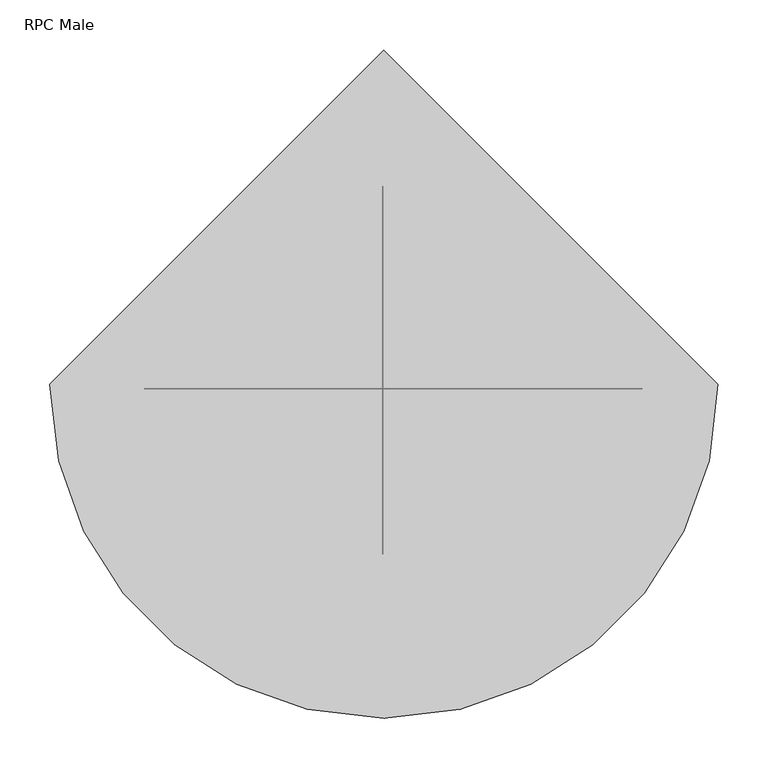
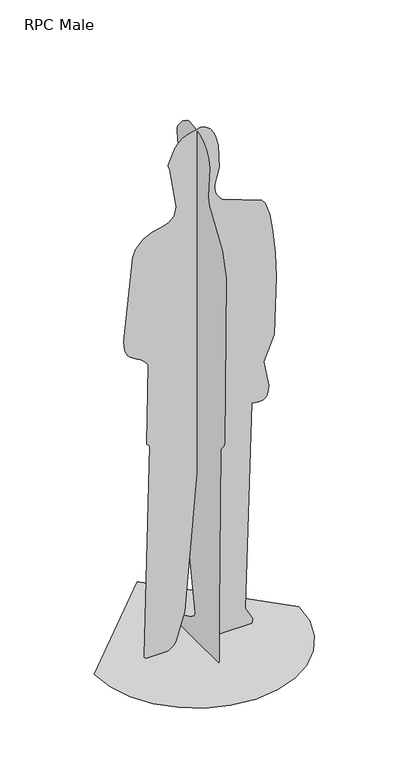
"""IFC4 building model written with IfcOpenShell, lengths in millimetres: proxy geometry, RPC Male : Dwayne."""

import ifcopenshell
import ifcopenshell.guid

model = None  # the IFC model being written
_history = None  # IfcOwnerHistory: only IFC2X3 demands one
_inside = {}  # id of a spatial element -> (the spatial element, [elements in it])
_under = {}  # id of a project, library or spatial element -> (it, [spatial elements below it])
_declared = {}  # id of a project -> (the project, [libraries it declares])
_typed = {}  # id of a type object -> (the type object, [elements of that type])
_made_of = {}  # id of a material, layer set ... -> (it, [elements and type objects made of it])


def new_model(schema):
    """Start an empty IFC model of exactly this schema.

    Asked for "IFC4X3", IfcOpenShell would pick the latest addendum, in which some entities
    have other attributes; the version numbers below select the first issue.
    IFC2X3 requires an IfcOwnerHistory on every rooted entity: one is made here for all.
    """
    global model, _history
    if schema == "IFC4X3":
        model = ifcopenshell.file(schema_version=(4, 3, 0, 0))
    else:
        model = ifcopenshell.file(schema=schema)
    _inside.clear()
    _under.clear()
    _declared.clear()
    _typed.clear()
    _made_of.clear()
    _history = None
    if model.schema == "IFC2X3":
        org = make("IfcOrganization", Name="unknown")
        user = make(
            "IfcPersonAndOrganization",
            ThePerson=make("IfcPerson", FamilyName="unknown"),
            TheOrganization=org,
        )
        app = make(
            "IfcApplication",
            ApplicationDeveloper=org,
            Version="unknown",
            ApplicationFullName="unknown",
            ApplicationIdentifier="unknown",
        )
        _history = make(
            "IfcOwnerHistory",
            OwningUser=user,
            OwningApplication=app,
            ChangeAction="ADDED",
            CreationDate=0,
        )
    return model


def make(cls, **values):
    """One entity of the class cls with the attributes given. An attribute that is None is left unset."""
    return model.create_entity(
        cls, **{name: value for name, value in values.items() if value is not None}
    )


def rooted(cls, **values):
    """An entity with a GlobalId (a new one), such as an element, a storey or a relation."""
    return make(cls, GlobalId=ifcopenshell.guid.new(), OwnerHistory=_history, **values)


def si_unit(unit_type, name, prefix=None):
    """IfcSIUnit, for example si_unit("LENGTHUNIT", "METRE", prefix="MILLI")."""
    return make("IfcSIUnit", UnitType=unit_type, Prefix=prefix, Name=name)


def assignment(units):
    """IfcUnitAssignment: the units of a project."""
    return None if units is None else make("IfcUnitAssignment", Units=units)


def point(xyz):
    """IfcCartesianPoint."""
    return None if xyz is None else make("IfcCartesianPoint", Coordinates=xyz)


def direction(xyz):
    """IfcDirection."""
    return None if xyz is None else make("IfcDirection", DirectionRatios=xyz)


def frame(location, z_axis=None, x_axis=None):
    """IfcAxis2Placement3D, a coordinate frame: its origin and axes. An axis left out is left unset."""
    return make(
        "IfcAxis2Placement3D",
        Location=point(location),
        Axis=direction(z_axis),
        RefDirection=direction(x_axis),
    )


def origin():
    """The frame at (0, 0, 0) with its axes left unset."""
    return frame((0.0, 0.0, 0.0))


def place(relative_to, where):
    """IfcLocalPlacement: puts the frame where relative to a parent placement (None: the world)."""
    return make(
        "IfcLocalPlacement", PlacementRelTo=relative_to, RelativePlacement=where
    )


def context(
    kind, dimensions, precision=None, world=None, true_north=None, identifier=None
):
    """IfcGeometricRepresentationContext, for example the 3D "Model" context."""
    return make(
        "IfcGeometricRepresentationContext",
        ContextIdentifier=identifier,
        ContextType=kind,
        CoordinateSpaceDimension=dimensions,
        Precision=precision,
        WorldCoordinateSystem=world,
        TrueNorth=true_north,
    )


def project(units=None, contexts=None):
    """IfcProject with its units and contexts."""
    return rooted(
        "IfcProject",
        Name="project",
        RepresentationContexts=contexts,
        UnitsInContext=assignment(units),
    )


def spatial(cls, under=None, at=None, **own):
    """A site, building, storey or space (cls), placed at a placement, below another one or the project."""
    s = rooted(cls, ObjectPlacement=at, **own)
    if under is not None:
        _under.setdefault(under.id(), (under, []))[1].append(s)
    return s


def point_list(points):
    """IfcCartesianPointList2D or 3D."""
    cls = (
        "IfcCartesianPointList2D" if len(points[0]) == 2 else "IfcCartesianPointList3D"
    )
    return make(cls, CoordList=points)


def triangles(points, corners, closed=None, point_numbers=None):
    """IfcTriangulatedFaceSet: each triangle names its three corners, points numbered from 1."""
    return make(
        "IfcTriangulatedFaceSet",
        Coordinates=point_list(points),
        Closed=closed,
        CoordIndex=corners,
        PnIndex=point_numbers,
    )


def shape(context_of_items, identifier, shape_type, items):
    """IfcShapeRepresentation: the items that make up one representation, for example the "Body"."""
    return make(
        "IfcShapeRepresentation",
        ContextOfItems=context_of_items,
        RepresentationIdentifier=identifier,
        RepresentationType=shape_type,
        Items=items,
    )


def source(mapping_origin, context_of_items, identifier, shape_type, items):
    """IfcRepresentationMap: a shape defined once, which mapped items show again and again."""
    return make(
        "IfcRepresentationMap",
        MappingOrigin=mapping_origin,
        MappedRepresentation=shape(context_of_items, identifier, shape_type, items),
    )


def transform(
    local_origin,
    x_axis=None,
    y_axis=None,
    z_axis=None,
    scale=None,
    scale2=None,
    scale3=None,
    uniform=True,
):
    """IfcCartesianTransformationOperator3D, or its non-uniform kind. x_axis, y_axis, z_axis: its Axis1, 2, 3."""
    if uniform:
        return make(
            "IfcCartesianTransformationOperator3D",
            Axis1=direction(x_axis),
            Axis2=direction(y_axis),
            LocalOrigin=point(local_origin),
            Scale=scale,
            Axis3=direction(z_axis),
        )
    return make(
        "IfcCartesianTransformationOperator3DnonUniform",
        Axis1=direction(x_axis),
        Axis2=direction(y_axis),
        LocalOrigin=point(local_origin),
        Scale=scale,
        Axis3=direction(z_axis),
        Scale2=scale2,
        Scale3=scale3,
    )


def mapped(mapping_source, mapping_target):
    """IfcMappedItem: shows the shape of a source again, moved by a transform."""
    return make(
        "IfcMappedItem", MappingSource=mapping_source, MappingTarget=mapping_target
    )


def made_of(thing, what):
    """Note that an element or type object is made of a material, layer set ...; save() writes the relation."""
    if what is not None:
        _made_of.setdefault(what.id(), (what, []))[1].append(thing)
    return thing


def element(
    cls,
    number,
    at=None,
    inside=None,
    cuts=None,
    type_object=None,
    material=None,
    context=None,
    identifier="Body",
    shape_type=None,
    held_by="IfcProductDefinitionShape",
    body=None,
    shapes=None,
    **own,
):
    """One element of the class cls, such as IfcWall. Its Tag is "e" and its number.

    at: its placement. inside: the storey or other place that contains it. cuts: it is an
    opening in that element (IfcRelVoidsElement). A single representation is given by context,
    identifier, shape_type and body (its items); several are given by shapes. held_by: the class
    of the entity that holds the representations. save() writes the other relations.
    """
    e = rooted(cls, Tag="e%d" % number, ObjectPlacement=at, **own)
    if body is not None:
        shapes = [shape(context, identifier, shape_type, body)]
    if shapes is not None:
        e.Representation = make(held_by, Representations=shapes)
    if inside is not None:
        _inside.setdefault(inside.id(), (inside, []))[1].append(e)
    if cuts is not None:
        rooted(
            "IfcRelVoidsElement", RelatingBuildingElement=cuts, RelatedOpeningElement=e
        )
    if type_object is not None:
        _typed.setdefault(type_object.id(), (type_object, []))[1].append(e)
    return made_of(e, material)


def aggregate(whole, parts):
    """IfcRelAggregates: a whole, such as a stair, and the parts it consists of."""
    return rooted("IfcRelAggregates", RelatingObject=whole, RelatedObjects=parts)


def save(model, path):
    """Write the relations noted so far, then the file.

    IfcRelAggregates (storeys below a building ...), IfcRelContainedInSpatialStructure (elements
    in a storey), IfcRelDefinesByType, IfcRelAssociatesMaterial and IfcRelDeclares: one each for
    every whole, place, type object, material and project.
    """
    for whole, parts in _under.values():
        aggregate(whole, parts)
    for where, things in _inside.values():
        rooted(
            "IfcRelContainedInSpatialStructure",
            RelatedElements=things,
            RelatingStructure=where,
        )
    for kind, things in _typed.values():
        rooted("IfcRelDefinesByType", RelatedObjects=things, RelatingType=kind)
    for what, things in _made_of.values():
        rooted("IfcRelAssociatesMaterial", RelatedObjects=things, RelatingMaterial=what)
    for by, libraries in _declared.values():
        rooted("IfcRelDeclares", RelatingContext=by, RelatedDefinitions=libraries)
    model.write(path)


def rpc_male_e00c4429(model_context):
    return source(origin(), model_context, "Body", "Tessellation", [
        triangles([(-180.7519758, -4.45e-05, 5.61e-05), (-184.2427693, -8.8e-06, 2.7953145), (-186.1721755, 1.66e-05, 5.8375002), (-186.8316374, 3.35e-05, 9.127569), (-168.2846227, 8.5e-06, 733.0652109), (-173.8813015, 8.5e-06, 735.2240908), (-177.6698602, 8.1e-06, 740.93319), (-174.1985423, -8.1e-06, 1013.6682867), (-179.591309, -8.8e-06, 1024.1651751), (-188.0395216, -9.6e-06, 1032.7759867), (-198.5267085, -9.9e-06, 1040.1126028), (-210.0363257, -1.03e-05, 1046.7864687), (-221.5520472, -1.07e-05, 1053.4092476), (-232.0572199, -1.1e-05, 1060.5929661), (-240.5353907, -1.14e-05, 1068.9488514), (-245.9518842, -1.21e-05, 1078.9880642), (-249.7386988, -1.29e-05, 1091.9821838), (-252.1552483, -1.4e-05, 1106.9298906), (-253.4607645, -1.47e-05, 1122.8295742), (-224.2188539, -3.16e-05, 1405.054644), (-213.7949444, -3.31e-05, 1430.2019463), (-189.1319694, -3.46e-05, 1456.0842327), (-160.624934, -3.53e-05, 1468.8737137), (-131.9229886, -3.57e-05, 1475.6378357), (-106.6752928, -3.64e-05, 1483.4436092), (-88.5310242, -3.71e-05, 1499.3593529), (-81.1392697, -3.9e-05, 1530.4516411), (-102.942045, -4.71e-05, 1666.4696468), (-107.9472446, -4.78e-05, 1679.2650867), (-108.1474504, -4.82e-05, 1680.5741638), (-107.984815, -4.82e-05, 1682.7587688), (-107.5268306, -4.82e-05, 1685.5190655), (-106.840944, -4.86e-05, 1688.5553627), (-86.6409052, -5.11e-05, 1733.0902897), (-74.2774293, -5.19e-05, 1747.7183212), (-59.5121605, -5.26e-05, 1759.6594528), (-42.363121, -5.33e-05, 1768.7777916), (-0.9855255, -5.37e-05, 1777.9990311), (15.8808757, -5.33e-05, 1772.5528519), (29.1619555, -5.26e-05, 1761.5639877), (39.2640369, -5.19e-05, 1747.0962662), (46.5934632, -5.08e-05, 1731.2140961), (56.009163, -4.89e-05, 1695.7207684), (59.1639487, -4.41e-05, 1618.2087845), (44.4858339, -4.12e-05, 1564.7278919), (44.3096682, -4.05e-05, 1551.1862766), (46.5532813, -3.94e-05, 1537.9279289), (51.2886345, -3.86e-05, 1525.4359589), (58.5876575, -3.83e-05, 1514.1926044), (68.5223164, -3.75e-05, 1504.6808304), (198.4030241, -3.46e-05, 1454.5808361), (210.7095586, -3.38e-05, 1440.8296406), (224.9005892, -3.13e-05, 1397.8447643), (235.5369131, -2.72e-05, 1333.6069702), (242.7580384, -2.28e-05, 1256.1532677), (246.7032373, -1.77e-05, 1173.5211021), (240.2781571, -5.9e-06, 974.9290089), (206.081389, -1.1e-06, 891.6222479), (221.1961823, 4e-06, 805.6633232), (220.4650678, 5.1e-06, 788.6200321), (214.9948893, 6.3e-06, 771.8045614), (210.3552016, 6.6e-06, 765.7300776), (204.1668257, 6.6e-06, 762.0919275), (196.8959759, 7e-06, 760.3982082), (189.0090118, 7e-06, 760.1573799), (180.9721295, 7e-06, 760.8774668), (173.2515615, 6.6e-06, 762.0669291), (166.3135766, 6.6e-06, 763.2339363), (144.8011179, 4.49e-05, 59.4752896), (168.6275342, 4.74e-05, 15.3365843), (166.1985945, -4.45e-05, 5.61e-05), (66.1332089, -4.45e-05, 5.61e-05), (49.8425018, -1.03e-05, 3.9765591), (39.0246256, 1.36e-05, 14.0353), (32.5983009, 2.91e-05, 28.3297116), (-2.7441046, 9.2e-06, 720.0458748), (-54.0725034, 1.03e-05, 117.9433278), (-81.3720135, -2.13e-05, 28.0047427), (-85.5237041, -2.69e-05, 19.9172686), (-91.2433859, -3.27e-05, 12.5691172), (-99.2451413, -3.86e-05, 5.9378887), (-110.2431982, -4.45e-05, 5.61e-05), (-13.8237406, -127.6718764, 9.9621145), (-13.8237974, -127.2617633, 182.0842528), (-13.8237815, -135.2635732, 744.8695776), (-13.8237815, -136.4149928, 748.3460369), (-13.8237815, -139.3954704, 752.5736132), (-13.8237815, -143.4944026, 757.5058702), (-13.8237815, -148.0010861, 763.0962994), (-13.8237815, -152.2049901, 769.2983917), (-13.8237792, -155.3953659, 776.0656385), (-13.8237792, -156.8616281, 783.3516764), (-13.8237622, -165.9465024, 1358.6137287), (-13.8237599, -143.2743216, 1442.0927902), (-13.8237576, -71.1145501, 1552.8585583), (-13.8237576, -64.3401725, 1580.5206779), (-13.8237542, -73.5344014, 1684.7952724), (-13.8237531, -67.2131212, 1712.2161278), (-13.8237531, -55.241223, 1734.9070393), (-13.8237531, -37.9260212, 1752.7537697), (-13.8237531, -15.5748771, 1765.6426632), (-13.8237531, 11.5049084, 1773.4593372), (-13.8237531, 43.0059914, 1776.090136), (-13.8237531, 55.0860226, 1772.9164925), (-13.8237542, 79.7038559, 1756.3218658), (-13.8237554, 107.4896145, 1722.3477768), (-13.8237554, 111.5711695, 1713.01012), (-13.8237554, 112.2229284, 1702.3019073), (-13.8237588, 99.0832235, 1611.9284992), (-13.8237588, 100.6007272, 1597.8206394), (-13.8237599, 96.755177, 1579.0656796), (-13.8237622, 31.1784566, 1488.4592915), (-13.8237735, 125.7984261, 1146.7472277), (-13.8237735, 134.1993577, 1137.675107), (-13.8237747, 184.2799037, 1119.3925747), (-13.8237747, 194.4649651, 1111.9394686), (-13.8237747, 201.1343255, 1100.3801451), (-13.8237769, 203.5508567, 1084.2058416), (-13.8237769, 200.9674025, 1068.9640394), (-13.8237769, 194.2820729, 1055.8707253), (-13.8237769, 184.3928146, 1046.1415226), (-13.8237769, 172.1978105, 1040.992709), (-13.8237769, 158.595007, 1041.6399078), (-13.8237769, 144.48246, 1049.299106), (-13.8237838, 123.0429529, 785.7648285), (-13.823786, 116.906318, 707.2429499), (-13.8237928, 10.2023683, 90.6853168), (-13.823794, 17.983895, 76.1481908), (-13.8237951, 35.4714404, 63.806743), (-13.8238042, 104.5965316, 31.8661463), (-13.8238053, 119.3344402, 20.2173661), (-13.8238076, 122.9915025, 6.7192091), (-13.8238042, 122.0607091, 4.3674998), (-13.8237894, 120.3451706, 2.3141478), (-13.8237724, 119.1853577, 1.4285653), (-13.8237474, 117.8199432, 0.6534771), (-13.8237099, 116.2458387, 5.61e-05), (-13.8237077, -124.501612, 0.0), (-348.4734607, 4.7230039, 0.0001684), (-339.5987117, -72.1961519, 0.0001684), (-314.3237646, -142.8340959, 5.61e-05), (-274.6722241, -205.1669827, 5.61e-05), (-222.6681673, -257.171094, 5.61e-05), (-160.3352533, -296.8225073, 5.61e-05), (-89.6973139, -322.097527, 5.61e-05), (-12.7781649, -330.972276, 5.61e-05), (64.1409886, -322.0975634, 5.61e-05), (134.7789371, -296.8225618, 5.61e-05), (197.1118239, -257.1710577, 5.61e-05), (249.1159897, -205.1670008, 5.61e-05), (288.7673667, -142.8340595, 5.61e-05), (314.0423864, -72.1960974, 0.0001684), (322.9171354, 4.7230331, 0.0001684), (-12.7782239, 340.4182474, 0.0001684)], [[70, 71, 72], [69, 70, 72], [69, 72, 73], [69, 73, 74], [69, 74, 75], [69, 75, 76], [68, 69, 76], [82, 1, 2], [82, 2, 3], [82, 3, 4], [81, 82, 4], [80, 81, 4], [79, 80, 4], [78, 79, 4], [77, 78, 4], [77, 4, 5], [76, 77, 5], [5, 6, 7], [76, 5, 7], [76, 7, 8], [68, 76, 8], [67, 68, 8], [66, 67, 8], [65, 66, 8], [64, 65, 8], [63, 64, 8], [62, 63, 8], [61, 62, 8], [60, 61, 8], [59, 60, 8], [58, 59, 8], [57, 58, 8], [56, 57, 8], [56, 8, 9], [55, 56, 9], [55, 9, 10], [54, 55, 10], [54, 10, 11], [53, 54, 11], [53, 11, 12], [52, 53, 12], [51, 52, 12], [50, 51, 12], [50, 12, 13], [50, 13, 14], [50, 14, 15], [50, 15, 16], [50, 16, 17], [50, 17, 18], [50, 18, 19], [50, 19, 20], [50, 20, 21], [50, 21, 22], [50, 22, 23], [50, 23, 24], [50, 24, 25], [50, 25, 26], [49, 50, 26], [48, 49, 26], [48, 26, 27], [47, 48, 27], [46, 47, 27], [45, 46, 27], [44, 45, 27], [44, 27, 28], [43, 44, 28], [42, 43, 28], [42, 28, 29], [42, 29, 30], [42, 30, 31], [42, 31, 32], [42, 32, 33], [42, 33, 34], [42, 34, 35], [42, 35, 36], [42, 36, 37], [41, 42, 37], [40, 41, 37], [40, 37, 38], [40, 38, 39], [137, 138, 83], [137, 83, 84], [136, 137, 84], [135, 136, 84], [130, 131, 132], [130, 132, 133], [130, 133, 134], [130, 134, 135], [122, 123, 124], [121, 122, 124], [120, 121, 124], [119, 120, 124], [118, 119, 124], [117, 118, 124], [116, 117, 124], [115, 116, 124], [114, 115, 124], [113, 114, 124], [106, 107, 108], [105, 106, 108], [104, 105, 108], [103, 104, 108], [102, 103, 108], [101, 102, 108], [100, 101, 108], [99, 100, 108], [98, 99, 108], [97, 98, 108], [97, 108, 109], [97, 109, 110], [97, 110, 111], [96, 97, 111], [95, 96, 111], [95, 111, 112], [94, 95, 112], [93, 94, 112], [93, 112, 113], [92, 93, 113], [92, 113, 124], [92, 124, 125], [91, 92, 125], [90, 91, 125], [89, 90, 125], [88, 89, 125], [87, 88, 125], [86, 87, 125], [86, 125, 126], [85, 86, 126], [85, 126, 127], [84, 85, 127], [84, 127, 128], [135, 84, 128], [135, 128, 129], [130, 135, 129], [153, 154, 139], [152, 153, 139], [152, 139, 140], [151, 152, 140], [151, 140, 141], [151, 141, 142], [150, 151, 142], [149, 150, 142], [149, 142, 143], [149, 143, 144], [149, 144, 145], [149, 145, 146], [149, 146, 147], [149, 147, 148]], closed=False),
    ])


if __name__ == "__main__":
    model = new_model("IFC4")
    model_context = context("Model", 3, world=origin())
    ifc_project = project(units=[si_unit("LENGTHUNIT", "METRE", prefix="MILLI")], contexts=[model_context])
    site = spatial("IfcSite", under=ifc_project)
    building = spatial("IfcBuilding", under=site)
    placement = place(None, origin())
    rpc_male_shape = rpc_male_e00c4429(model_context)
    element("IfcBuildingElementProxy", 1, Name="RPC Male : Dwayne", ObjectType="RPC Male : Dwayne", at=placement, inside=building, context=model_context, shape_type="MappedRepresentation", body=[
        mapped(rpc_male_shape, transform((0.0, 0.0, 0.0), x_axis=(1.0, 0.0, 0.0), y_axis=(0.0, 1.0, 0.0), z_axis=(0.0, 0.0, 1.0))),
    ])
    save(model, "model.ifc")

# Revit data of these elements
# Type "RPC Male : Dwayne"
#   built-in parameter 1005198 = "{2, 15},{22, RPC-8-G1AE-S4G0-CKUK-A},{1, 0},{1, 0},{2, 15},{1, 8},{5, Color},{1, 0},{1, 0},{3, 0.8},{3, 0.8},{3, 0.8},{1, 8},{7, BBoxMin},{1, 0},{1, 0},{1, 0},{1, 0},{1, 0},{1, 8},{7, BBoxMax},{1, 0},{1, 0},{1, 0},{1, 0},{1, 0},{2, 11},{9, RPCTypeId},{1, 0},{1, 0},{22, RPC-8-G1AE-S4G0-CKUK-A},{1, 6},{14, RPCPlantHeight},{1, 0},{1, 0},{7, 5.83333},{2, 11},{7, keyword},{1, 0},{1, 0},{45, :RPCs:People [Business-Hispanic]:Geometry:RPC},{2, 11},{8, category},{1, 0},{1, 0},{26, People [Business-Hispanic]},{2, 11},{12, LocalizedUID},{1, 0},{1, 0},{6, Dwayne},{2, 14},{6, Height},{1, 0},{1, 0},{7, 5.83333},{1, 2},{16, Cast Reflections},{1, 0},{1, 0},{1, 0},{1, 2},{6, Jitter},{1, 0},{1, 0},{1, 1},{1, 2},{9, Billboard},{1, 0},{1, 0},{1, 0},{1, 2},{12, Cast Shadows},{1, 0},{1, 0},{1, 1},{1, 2},{20, Apply Filter Effects},{1, 0},{1, 0},{1, 0},{2, 11},{28, Apply Filter Effects-Text-FC},{1, 0},{1, 0},{4, None},{21, assetlibrary_base.fbx},{1, 5},"
#   built-in parameter 1005195 = "RPC-8-G1AE-S4G0-CKUK-A"
#   Height = 0
